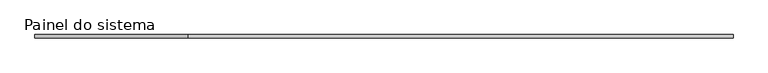
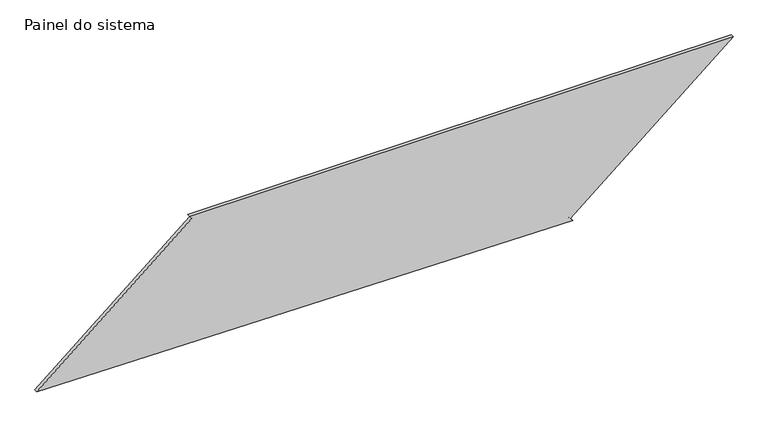
"""IFC4 building model written with IfcOpenShell, lengths in millimetres: plate geometry, Painel do sistema : Envidraçado."""

from ifc_helpers import new_model, si_unit, frame, origin, place, context, project, spatial, polyline, outline, extrude, source, transform, mapped, element, save


def painel_do_sistema_dad1f5aa(model_context):
    return source(origin(), model_context, "Body", "SweptSolid", [
        extrude(outline(polyline([(0.0, 1373.6700134), (19.2037959, 1357.6633203), (1012.0276234, 2548.7891861), (1012.0276234, -1430.2165437), (992.8238275, -1414.2098506), (47.1325024, -2548.7891861), (0.0, 1373.6700134)])), frame((0.0, 24.5, 0.0), z_axis=(0.0, 1.0, 0.0), x_axis=(0.0, 0.0, 1.0)), (0.0, 0.0, 1.0), 25.0),
    ])


if __name__ == "__main__":
    model = new_model("IFC4")
    model_context = context("Model", 3, world=origin())
    ifc_project = project(units=[si_unit("LENGTHUNIT", "METRE", prefix="MILLI")], contexts=[model_context])
    site = spatial("IfcSite", under=ifc_project)
    building = spatial("IfcBuilding", under=site)
    placement = place(None, origin())
    painel_do_sistema_shape = painel_do_sistema_dad1f5aa(model_context)
    element("IfcPlate", 1, ObjectType="Painel do sistema : Envidraçado", at=placement, inside=building, context=model_context, shape_type="MappedRepresentation", body=[
        mapped(painel_do_sistema_shape, transform((0.0, 0.0, 0.0), x_axis=(1.0, 0.0, 0.0), y_axis=(0.0, 1.0, 0.0), z_axis=(0.0, 0.0, 1.0))),
    ])
    save(model, "model.ifc")

# Revit data of these elements
# Type "Painel do sistema : Envidraçado"
#   Construction Type Id = "GSP4R"
#   Analytic Construction = "Vidraça única Pilkington 1/8 pol"
#   Visual Light Transmittance = 0.9
#   Solar Heat Gain Coefficient = 0.86
#   Heat Transfer Coefficient (U) = 6.7069 W/(m²·K)
# Element 1 (IfcPlate, "Painel do sistema : Envidraçado")
#   Materials on its faces: "Vidro"
# Materials
#   "Vidro": class "Vidro", colour RGB 0 128 192, transparency 0.9, Description = "Vidro de sílica", Cost = 0
